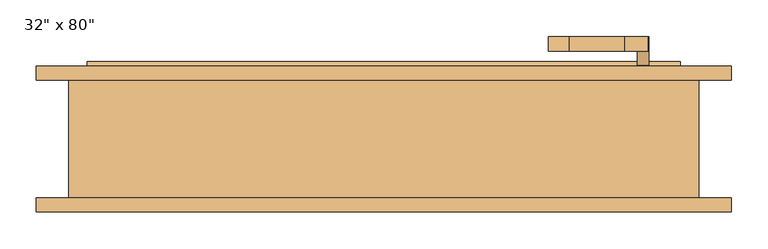
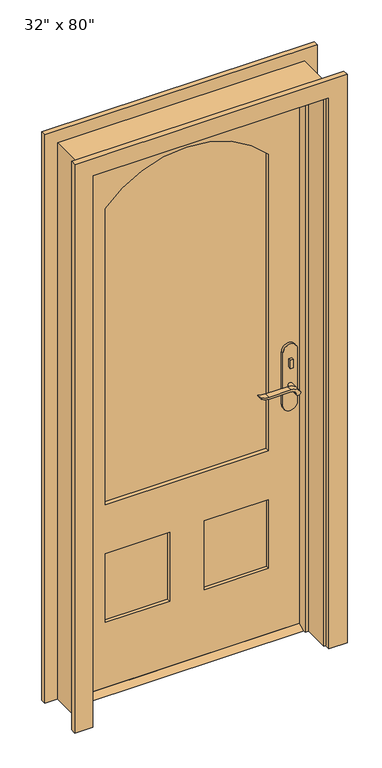
"""IFC4 building model written with IfcOpenShell, lengths in millimetres: door geometry."""

import ifcopenshell
import ifcopenshell.guid

model = None  # the IFC model being written
_history = None  # IfcOwnerHistory: only IFC2X3 demands one
_inside = {}  # id of a spatial element -> (the spatial element, [elements in it])
_under = {}  # id of a project, library or spatial element -> (it, [spatial elements below it])
_declared = {}  # id of a project -> (the project, [libraries it declares])
_typed = {}  # id of a type object -> (the type object, [elements of that type])
_made_of = {}  # id of a material, layer set ... -> (it, [elements and type objects made of it])


def new_model(schema):
    """Start an empty IFC model of exactly this schema.

    Asked for "IFC4X3", IfcOpenShell would pick the latest addendum, in which some entities
    have other attributes; the version numbers below select the first issue.
    IFC2X3 requires an IfcOwnerHistory on every rooted entity: one is made here for all.
    """
    global model, _history
    if schema == "IFC4X3":
        model = ifcopenshell.file(schema_version=(4, 3, 0, 0))
    else:
        model = ifcopenshell.file(schema=schema)
    _inside.clear()
    _under.clear()
    _declared.clear()
    _typed.clear()
    _made_of.clear()
    _history = None
    if model.schema == "IFC2X3":
        org = make("IfcOrganization", Name="unknown")
        user = make(
            "IfcPersonAndOrganization",
            ThePerson=make("IfcPerson", FamilyName="unknown"),
            TheOrganization=org,
        )
        app = make(
            "IfcApplication",
            ApplicationDeveloper=org,
            Version="unknown",
            ApplicationFullName="unknown",
            ApplicationIdentifier="unknown",
        )
        _history = make(
            "IfcOwnerHistory",
            OwningUser=user,
            OwningApplication=app,
            ChangeAction="ADDED",
            CreationDate=0,
        )
    return model


def make(cls, **values):
    """One entity of the class cls with the attributes given. An attribute that is None is left unset."""
    return model.create_entity(
        cls, **{name: value for name, value in values.items() if value is not None}
    )


def rooted(cls, **values):
    """An entity with a GlobalId (a new one), such as an element, a storey or a relation."""
    return make(cls, GlobalId=ifcopenshell.guid.new(), OwnerHistory=_history, **values)


def si_unit(unit_type, name, prefix=None):
    """IfcSIUnit, for example si_unit("LENGTHUNIT", "METRE", prefix="MILLI")."""
    return make("IfcSIUnit", UnitType=unit_type, Prefix=prefix, Name=name)


def assignment(units):
    """IfcUnitAssignment: the units of a project."""
    return None if units is None else make("IfcUnitAssignment", Units=units)


def point(xyz):
    """IfcCartesianPoint."""
    return None if xyz is None else make("IfcCartesianPoint", Coordinates=xyz)


def direction(xyz):
    """IfcDirection."""
    return None if xyz is None else make("IfcDirection", DirectionRatios=xyz)


def frame(location, z_axis=None, x_axis=None):
    """IfcAxis2Placement3D, a coordinate frame: its origin and axes. An axis left out is left unset."""
    return make(
        "IfcAxis2Placement3D",
        Location=point(location),
        Axis=direction(z_axis),
        RefDirection=direction(x_axis),
    )


def frame_2d(location, x_axis=None):
    """IfcAxis2Placement2D, a coordinate frame in the plane: its origin and x axis."""
    return make(
        "IfcAxis2Placement2D", Location=point(location), RefDirection=direction(x_axis)
    )


def origin():
    """The frame at (0, 0, 0) with its axes left unset."""
    return frame((0.0, 0.0, 0.0))


def place(relative_to, where):
    """IfcLocalPlacement: puts the frame where relative to a parent placement (None: the world)."""
    return make(
        "IfcLocalPlacement", PlacementRelTo=relative_to, RelativePlacement=where
    )


def context(
    kind, dimensions, precision=None, world=None, true_north=None, identifier=None
):
    """IfcGeometricRepresentationContext, for example the 3D "Model" context."""
    return make(
        "IfcGeometricRepresentationContext",
        ContextIdentifier=identifier,
        ContextType=kind,
        CoordinateSpaceDimension=dimensions,
        Precision=precision,
        WorldCoordinateSystem=world,
        TrueNorth=true_north,
    )


def project(units=None, contexts=None):
    """IfcProject with its units and contexts."""
    return rooted(
        "IfcProject",
        Name="project",
        RepresentationContexts=contexts,
        UnitsInContext=assignment(units),
    )


def spatial(cls, under=None, at=None, **own):
    """A site, building, storey or space (cls), placed at a placement, below another one or the project."""
    s = rooted(cls, ObjectPlacement=at, **own)
    if under is not None:
        _under.setdefault(under.id(), (under, []))[1].append(s)
    return s


def polyline(points):
    """IfcPolyline through the points."""
    return make("IfcPolyline", Points=[point(p) for p in points])


def circle_curve(where, radius):
    """IfcCircle in the frame where."""
    return make("IfcCircle", Position=where, Radius=radius)


def trimmed(basis, trim1, trim2, sense, master):
    """IfcTrimmedCurve: the piece of a basis curve between two trims."""
    return make(
        "IfcTrimmedCurve",
        BasisCurve=basis,
        Trim1=trim1,
        Trim2=trim2,
        SenseAgreement=sense,
        MasterRepresentation=master,
    )


def segment(curve, same_sense, transition):
    """IfcCompositeCurveSegment."""
    return make(
        "IfcCompositeCurveSegment",
        Transition=transition,
        SameSense=same_sense,
        ParentCurve=curve,
    )


def composite_curve(segments, self_intersect=None):
    """IfcCompositeCurve: segments joined end to end."""
    return make("IfcCompositeCurve", Segments=segments, SelfIntersect=self_intersect)


def outline(outer, holes=None, kind="AREA"):
    """IfcArbitraryClosedProfileDef: a profile drawn as a closed curve; with holes, ...WithVoids."""
    if holes is None:
        return make("IfcArbitraryClosedProfileDef", ProfileType=kind, OuterCurve=outer)
    return make(
        "IfcArbitraryProfileDefWithVoids",
        ProfileType=kind,
        OuterCurve=outer,
        InnerCurves=holes,
    )


def extrude(swept, where, along, depth):
    """IfcExtrudedAreaSolid: the profile swept, set in the frame where, extruded along a direction by depth."""
    return make(
        "IfcExtrudedAreaSolid",
        SweptArea=swept,
        Position=where,
        ExtrudedDirection=direction(along),
        Depth=depth,
    )


def faces_of(points, faces, orient=None, outer=None):
    """IfcFace entities. A face is a list of loops; a loop is a list of indices into points, from 0.

    orient and outer hold one flag for each loop. By default every Orientation is true, the
    first loop of a face is its IfcFaceOuterBound and the others are IfcFaceBound.
    """
    made = []
    for i, loops in enumerate(faces):
        bounds = []
        for j, loop in enumerate(loops):
            is_outer = j == 0 if outer is None else outer[i][j]
            bounds.append(
                make(
                    "IfcFaceOuterBound" if is_outer else "IfcFaceBound",
                    Bound=make("IfcPolyLoop", Polygon=[points[k] for k in loop]),
                    Orientation=True if orient is None else orient[i][j],
                )
            )
        made.append(make("IfcFace", Bounds=bounds))
    return made


def faceted_brep(points, faces, orient=None, outer=None, voids=None):
    """IfcFacetedBrep: a solid bounded by flat faces; with voids (closed shells), ...WithVoids."""
    shared = [point(p) for p in points]
    hull = make("IfcClosedShell", CfsFaces=faces_of(shared, faces, orient, outer))
    if voids is None:
        return make("IfcFacetedBrep", Outer=hull)
    return make(
        "IfcFacetedBrepWithVoids",
        Outer=hull,
        Voids=[
            make(cls, CfsFaces=faces_of(shared, fs, o, b)) for cls, fs, o, b in voids
        ],
    )


def shape(context_of_items, identifier, shape_type, items):
    """IfcShapeRepresentation: the items that make up one representation, for example the "Body"."""
    return make(
        "IfcShapeRepresentation",
        ContextOfItems=context_of_items,
        RepresentationIdentifier=identifier,
        RepresentationType=shape_type,
        Items=items,
    )


def source(mapping_origin, context_of_items, identifier, shape_type, items):
    """IfcRepresentationMap: a shape defined once, which mapped items show again and again."""
    return make(
        "IfcRepresentationMap",
        MappingOrigin=mapping_origin,
        MappedRepresentation=shape(context_of_items, identifier, shape_type, items),
    )


def transform(
    local_origin,
    x_axis=None,
    y_axis=None,
    z_axis=None,
    scale=None,
    scale2=None,
    scale3=None,
    uniform=True,
):
    """IfcCartesianTransformationOperator3D, or its non-uniform kind. x_axis, y_axis, z_axis: its Axis1, 2, 3."""
    if uniform:
        return make(
            "IfcCartesianTransformationOperator3D",
            Axis1=direction(x_axis),
            Axis2=direction(y_axis),
            LocalOrigin=point(local_origin),
            Scale=scale,
            Axis3=direction(z_axis),
        )
    return make(
        "IfcCartesianTransformationOperator3DnonUniform",
        Axis1=direction(x_axis),
        Axis2=direction(y_axis),
        LocalOrigin=point(local_origin),
        Scale=scale,
        Axis3=direction(z_axis),
        Scale2=scale2,
        Scale3=scale3,
    )


def mapped(mapping_source, mapping_target):
    """IfcMappedItem: shows the shape of a source again, moved by a transform."""
    return make(
        "IfcMappedItem", MappingSource=mapping_source, MappingTarget=mapping_target
    )


def made_of(thing, what):
    """Note that an element or type object is made of a material, layer set ...; save() writes the relation."""
    if what is not None:
        _made_of.setdefault(what.id(), (what, []))[1].append(thing)
    return thing


def element(
    cls,
    number,
    at=None,
    inside=None,
    cuts=None,
    type_object=None,
    material=None,
    context=None,
    identifier="Body",
    shape_type=None,
    held_by="IfcProductDefinitionShape",
    body=None,
    shapes=None,
    **own,
):
    """One element of the class cls, such as IfcWall. Its Tag is "e" and its number.

    at: its placement. inside: the storey or other place that contains it. cuts: it is an
    opening in that element (IfcRelVoidsElement). A single representation is given by context,
    identifier, shape_type and body (its items); several are given by shapes. held_by: the class
    of the entity that holds the representations. save() writes the other relations.
    """
    e = rooted(cls, Tag="e%d" % number, ObjectPlacement=at, **own)
    if body is not None:
        shapes = [shape(context, identifier, shape_type, body)]
    if shapes is not None:
        e.Representation = make(held_by, Representations=shapes)
    if inside is not None:
        _inside.setdefault(inside.id(), (inside, []))[1].append(e)
    if cuts is not None:
        rooted(
            "IfcRelVoidsElement", RelatingBuildingElement=cuts, RelatedOpeningElement=e
        )
    if type_object is not None:
        _typed.setdefault(type_object.id(), (type_object, []))[1].append(e)
    return made_of(e, material)


def aggregate(whole, parts):
    """IfcRelAggregates: a whole, such as a stair, and the parts it consists of."""
    return rooted("IfcRelAggregates", RelatingObject=whole, RelatedObjects=parts)


def save(model, path):
    """Write the relations noted so far, then the file.

    IfcRelAggregates (storeys below a building ...), IfcRelContainedInSpatialStructure (elements
    in a storey), IfcRelDefinesByType, IfcRelAssociatesMaterial and IfcRelDeclares: one each for
    every whole, place, type object, material and project.
    """
    for whole, parts in _under.values():
        aggregate(whole, parts)
    for where, things in _inside.values():
        rooted(
            "IfcRelContainedInSpatialStructure",
            RelatedElements=things,
            RelatingStructure=where,
        )
    for kind, things in _typed.values():
        rooted("IfcRelDefinesByType", RelatedObjects=things, RelatingType=kind)
    for what, things in _made_of.values():
        rooted("IfcRelAssociatesMaterial", RelatedObjects=things, RelatingMaterial=what)
    for by, libraries in _declared.values():
        rooted("IfcRelDeclares", RelatingContext=by, RelatedDefinitions=libraries)
    model.write(path)


def door_3993ae6d(model_context):
    return source(origin(), model_context, "Body", "SolidModel", [
        extrude(outline(polyline([(42.8625, 12.7), (77.7875, 12.7), (103.1875, 0.0), (17.4625, 0.0), (42.8625, 12.7)])), frame((-406.4, 0.0, 0.0), z_axis=(1.0, 0.0, 0.0), x_axis=(0.0, 1.0, 0.0)), (0.0, 0.0, 1.0), 812.8),
        extrude(outline(polyline([(360.6, 22.8625), (350.6, 22.8625), (350.6, 32.8625), (360.6, 32.8625), (360.6, 22.8625)])), frame((0.0, 0.0, 981.9), z_axis=(0.0, 0.0, 1.0), x_axis=(1.0, 0.0, 0.0)), (0.0, 0.0, 1.0), 30.0),
        extrude(outline(composite_curve([segment(trimmed(circle_curve(frame_2d((996.9, 355.6)), 8.0), [point((996.9, 347.6))], [point((996.9, 363.6))], False, "CARTESIAN"), True, "CONTINUOUS"), segment(trimmed(circle_curve(frame_2d((996.9, 355.6)), 8.0), [point((996.9, 363.6))], [point((996.9, 347.6))], False, "CARTESIAN"), True, "CONTINUOUS")], self_intersect=False)), frame((0.0, 87.7875, 0.0), z_axis=(0.0, 1.0, 0.0), x_axis=(0.0, 0.0, 1.0)), (0.0, 0.0, 1.0), 10.0),
        extrude(outline(composite_curve([segment(trimmed(circle_curve(frame_2d((897.1555521, 331.9324871)), 37.2832219), [point((919.0523287, 362.1081363))], [point((934.4, 330.2325667))], False, "CARTESIAN"), True, "CONTINUOUS"), segment(polyline([(934.4, 330.2325667), (934.4, 253.9564091)]), True, "CONTINUOUS"), segment(trimmed(circle_curve(frame_2d((1017.6850638, 254.0227909)), 83.2850902), [point((934.4, 253.9564091))], [point((939.4, 225.6))], True, "CARTESIAN"), True, "CONTINUOUS"), segment(polyline([(939.4, 225.6), (936.6135558, 225.6)]), True, "CONTINUOUS"), segment(trimmed(circle_curve(frame_2d((986.6709207, 257.5396612)), 59.3791355), [point((936.6135558, 225.6))], [point((927.4, 253.9564091))], False, "CARTESIAN"), True, "CONTINUOUS"), segment(polyline([(927.4, 253.9564091), (927.4, 330.2138099)]), True, "CONTINUOUS"), segment(trimmed(circle_curve(frame_2d((909.2738613, 330.2138099)), 18.1261387), [point((927.4, 330.2138099))], [point((914.4, 347.6))], True, "CARTESIAN"), True, "CONTINUOUS"), segment(trimmed(circle_curve(frame_2d((914.4, 355.6)), 8.0), [point((914.4, 347.6))], [point((919.0523287, 362.1081363))], False, "CARTESIAN"), True, "CONTINUOUS")], self_intersect=False)), frame((0.0, -17.1375, 0.0), z_axis=(0.0, 1.0, 0.0), x_axis=(0.0, 0.0, 1.0)), (0.0, 0.0, 1.0), 20.0),
        extrude(outline(composite_curve([segment(trimmed(circle_curve(frame_2d((914.4, 355.6)), 8.0), [point((914.3999903, 347.6))], [point((919.0523287, 362.1081363))], False, "CARTESIAN"), True, "CONTINUOUS"), segment(trimmed(circle_curve(frame_2d((897.1555521, 331.9324871)), 37.2832219), [point((919.0523287, 362.1081363))], [point((934.4, 330.2325667))], False, "CARTESIAN"), True, "CONTINUOUS"), segment(polyline([(934.4, 330.2325667), (934.4, 253.9564091)]), True, "CONTINUOUS"), segment(trimmed(circle_curve(frame_2d((1017.6850638, 254.0227909)), 83.2850902), [point((934.4, 253.9564091))], [point((939.4, 225.6))], True, "CARTESIAN"), True, "CONTINUOUS"), segment(polyline([(939.4, 225.6), (936.6135558, 225.6)]), True, "CONTINUOUS"), segment(trimmed(circle_curve(frame_2d((986.6709207, 257.5396612)), 59.3791355), [point((936.6135558, 225.6))], [point((927.4, 253.9564091))], False, "CARTESIAN"), True, "CONTINUOUS"), segment(polyline([(927.4, 253.9564091), (927.4, 330.2138122)]), True, "CONTINUOUS"), segment(trimmed(circle_curve(frame_2d((909.2738682, 330.2138122)), 18.1261318), [point((927.4, 330.2138122))], [point((914.3999903, 347.6))], True, "CARTESIAN"), True, "CONTINUOUS")], self_intersect=False)), frame((0.0, 117.7875, 0.0), z_axis=(0.0, 1.0, 0.0), x_axis=(0.0, 0.0, 1.0)), (0.0, 0.0, 1.0), 20.0),
        extrude(outline(composite_curve([segment(trimmed(circle_curve(frame_2d((914.4, 355.6)), 8.0), [point((914.4, 347.6))], [point((914.4, 363.6))], False, "CARTESIAN"), True, "CONTINUOUS"), segment(trimmed(circle_curve(frame_2d((914.4, 355.6)), 8.0), [point((914.4, 363.6))], [point((914.4, 347.6))], False, "CARTESIAN"), True, "CONTINUOUS")], self_intersect=False)), frame((0.0, 2.8625, 0.0), z_axis=(0.0, 1.0, 0.0), x_axis=(0.0, 0.0, 1.0)), (0.0, 0.0, 1.0), 30.0),
        extrude(outline(composite_curve([segment(trimmed(circle_curve(frame_2d((914.4, 355.6)), 8.0), [point((914.4, 347.6))], [point((914.4, 363.6))], False, "CARTESIAN"), True, "CONTINUOUS"), segment(trimmed(circle_curve(frame_2d((914.4, 355.6)), 8.0), [point((914.4, 363.6))], [point((914.4, 347.6))], False, "CARTESIAN"), True, "CONTINUOUS")], self_intersect=False)), frame((0.0, 87.7875, 0.0), z_axis=(0.0, 1.0, 0.0), x_axis=(0.0, 0.0, 1.0)), (0.0, 0.0, 1.0), 30.0),
        extrude(outline(composite_curve([segment(polyline([(844.4, 380.6), (1039.4, 380.6)]), True, "CONTINUOUS"), segment(trimmed(circle_curve(frame_2d((1039.4, 355.6)), 25.0), [point((1039.4, 380.6))], [point((1039.4, 330.6))], False, "CARTESIAN"), True, "CONTINUOUS"), segment(polyline([(1039.4, 330.6), (844.4, 330.6)]), True, "CONTINUOUS"), segment(trimmed(circle_curve(frame_2d((844.4, 355.6)), 25.0), [point((844.4, 330.6))], [point((844.4, 380.6))], False, "CARTESIAN"), True, "CONTINUOUS")], self_intersect=False)), frame((0.0, 32.8625, 0.0), z_axis=(0.0, 1.0, 0.0), x_axis=(0.0, 0.0, 1.0)), (0.0, 0.0, 1.0), 10.0),
        extrude(outline(composite_curve([segment(polyline([(844.4, 380.6), (1039.4, 380.6)]), True, "CONTINUOUS"), segment(trimmed(circle_curve(frame_2d((1039.4, 355.6)), 25.0), [point((1039.4, 380.6))], [point((1039.4, 330.6))], False, "CARTESIAN"), True, "CONTINUOUS"), segment(polyline([(1039.4, 330.6), (844.4, 330.6)]), True, "CONTINUOUS"), segment(trimmed(circle_curve(frame_2d((844.4, 355.6)), 25.0), [point((844.4, 330.6))], [point((844.4, 380.6))], False, "CARTESIAN"), True, "CONTINUOUS")], self_intersect=False)), frame((0.0, 77.7875, 0.0), z_axis=(0.0, 1.0, 0.0), x_axis=(0.0, 0.0, 1.0)), (0.0, 0.0, 1.0), 10.0),
        extrude(outline(polyline([(2032.0, -406.4), (12.7, -406.4), (12.7, 406.4), (2032.0, 406.4), (2032.0, -406.4)]), holes=[composite_curve([segment(polyline([(688.975, -285.75), (1784.35, -285.75)]), True, "CONTINUOUS"), segment(trimmed(circle_curve(frame_2d((1526.38125, 0.0)), 384.96875), [point((1784.35, -285.75))], [point((1784.35, 285.75))], True, "CARTESIAN"), True, "CONTINUOUS"), segment(polyline([(1784.35, 285.75), (688.975, 285.75), (688.975, -285.75)]), True, "CONTINUOUS")], self_intersect=False), polyline([(508.0, -60.325), (254.0, -60.325), (254.0, -285.75), (508.0, -285.75), (508.0, -60.325)]), polyline([(508.0, 285.75), (254.0, 285.75), (254.0, 60.325), (508.0, 60.325), (508.0, 285.75)])]), frame((0.0, 42.8625, 0.0), z_axis=(0.0, 1.0, 0.0), x_axis=(0.0, 0.0, 1.0)), (0.0, 0.0, 1.0), 34.925),
        faceted_brep([(431.8, 77.7875, 0.0), (431.8, -84.1375, 0.0), (406.4, -84.1375, 0.0), (406.4, 7.9375, 0.0), (393.7, 7.9375, 0.0), (393.7, 42.8625, 0.0), (406.4, 42.8625, 0.0), (406.4, 77.7875, 0.0), (431.8, 77.7875, 2057.4), (431.8, -84.1375, 2057.4), (-431.8, -84.1375, 2057.4), (-431.8, -84.1375, 0.0), (-406.4, -84.1375, 0.0), (-406.4, -84.1375, 2032.0), (406.4, -84.1375, 2032.0), (406.4, 7.9375, 2032.0), (-406.4, 7.9375, 2032.0), (-406.4, 7.9375, 0.0), (-393.7, 7.9375, 0.0), (-393.7, 7.9375, 2019.3), (393.7, 7.9375, 2019.3), (393.7, 42.8625, 2019.3), (-393.7, 42.8625, 2019.3), (-393.7, 42.8625, 0.0), (-406.4, 42.8625, 0.0), (-406.4, 42.8625, 2032.0), (406.4, 42.8625, 2032.0), (406.4, 77.7875, 2032.0), (-406.4, 77.7875, 2032.0), (-406.4, 77.7875, 0.0), (-431.8, 77.7875, 0.0), (-431.8, 77.7875, 2057.4)], [[[0, 1, 2, 3, 4, 5, 6, 7]], [[1, 0, 8, 9]], [[2, 1, 9, 10, 11, 12, 13, 14]], [[3, 2, 14, 15]], [[4, 3, 15, 16, 17, 18, 19, 20]], [[5, 4, 20, 21]], [[6, 5, 21, 22, 23, 24, 25, 26]], [[7, 6, 26, 27]], [[0, 7, 27, 28, 29, 30, 31, 8]], [[9, 8, 31, 10]], [[15, 14, 13, 16]], [[21, 20, 19, 22]], [[27, 26, 25, 28]], [[30, 29, 24, 23, 18, 17, 12, 11]], [[10, 31, 30, 11]], [[16, 13, 12, 17]], [[22, 19, 18, 23]], [[28, 25, 24, 29]]]),
        extrude(outline(polyline([(-60.325, 54.5041667), (-285.75, 54.5041667), (-285.75, 66.1458333), (-60.325, 66.1458333), (-60.325, 54.5041667)])), frame((0.0, 0.0, 254.0), z_axis=(0.0, 0.0, 1.0), x_axis=(1.0, 0.0, 0.0)), (0.0, 0.0, 1.0), 254.0),
        extrude(outline(polyline([(285.75, 54.5041667), (60.325, 54.5041667), (60.325, 66.1458333), (285.75, 66.1458333), (285.75, 54.5041667)])), frame((0.0, 0.0, 254.0), z_axis=(0.0, 0.0, 1.0), x_axis=(1.0, 0.0, 0.0)), (0.0, 0.0, 1.0), 254.0),
        extrude(outline(composite_curve([segment(polyline([(688.975, -285.75), (688.975, 285.75), (1784.35, 285.75)]), True, "CONTINUOUS"), segment(trimmed(circle_curve(frame_2d((1526.38125, 0.0)), 384.96875), [point((1784.35, 285.75))], [point((1784.35, -285.75))], False, "CARTESIAN"), True, "CONTINUOUS"), segment(polyline([(1784.35, -285.75), (688.975, -285.75)]), True, "CONTINUOUS")], self_intersect=False)), frame((0.0, 56.8325, 0.0), z_axis=(0.0, 1.0, 0.0), x_axis=(0.0, 0.0, 1.0)), (0.0, 0.0, 1.0), 6.985),
        extrude(outline(polyline([(0.0, -476.25), (0.0, -412.75), (2038.35, -412.75), (2038.35, 412.75), (0.0, 412.75), (0.0, 476.25), (2101.85, 476.25), (2101.85, -476.25), (0.0, -476.25)])), frame((0.0, -103.1875, 0.0), z_axis=(0.0, 1.0, 0.0), x_axis=(0.0, 0.0, 1.0)), (0.0, 0.0, 1.0), 19.05),
        extrude(outline(polyline([(0.0, -476.25), (0.0, -412.75), (2038.35, -412.75), (2038.35, 412.75), (0.0, 412.75), (0.0, 476.25), (2101.85, 476.25), (2101.85, -476.25), (0.0, -476.25)])), frame((0.0, 77.7875, 0.0), z_axis=(0.0, 1.0, 0.0), x_axis=(0.0, 0.0, 1.0)), (0.0, 0.0, 1.0), 19.05),
    ])


if __name__ == "__main__":
    model = new_model("IFC4")
    model_context = context("Model", 3, world=origin())
    ifc_project = project(units=[si_unit("LENGTHUNIT", "METRE", prefix="MILLI")], contexts=[model_context])
    site = spatial("IfcSite", under=ifc_project)
    building = spatial("IfcBuilding", under=site)
    placement = place(None, origin())
    door_shape = door_3993ae6d(model_context)
    element("IfcDoor", 1, ObjectType="Door-Exterior-Single-Entry-Half Arch Glass-Wood_Clad : 32\" x 80\"", at=placement, inside=building, context=model_context, shape_type="MappedRepresentation", body=[
        mapped(door_shape, transform((0.0, 0.0, 0.0), x_axis=(1.0, 0.0, 0.0), y_axis=(0.0, 1.0, 0.0), z_axis=(0.0, 0.0, 1.0))),
    ])
    save(model, "model.ifc")

# Revit data of these elements
# Type "Door-Exterior-Single-Entry-Half Arch Glass-Wood_Clad : 32\" x 80\""
#   Type Mark = "112"
#   COBie.Type.CreatedBy = "doug.wood@us.ibm.com"
#   COBie.Type.CreatedOn = "2016-04-14T02:07:24"
#   COBie.Type.Name = "Doors_Door-Exterior-Single-Entry-Half Arch Glass-Wood_Clad_32\" x 80\"_112"
#   COBie.Type.Category = "23-30 10 14 : Passage Doors by Material"
#   COBie.Type.Description = "Door-Exterior-Single-Entry-Half Arch Glass-Wood_Clad_32\" x 80\""
#   COBie.Type.Manufacturer = ""
#   COBie.Type.ModelNumber = ""
#   Assembly Code = "B2030100"
#   Analytic Construction = "French door, wood frame with single glass"
#   COBie.Type.ReplacementCost = 0
#   Threshold Offset [instance default] = 0' - 0 1/2"
#   Thickness = 0' - 1 3/8"
#   Thermal Resistance (R) = 0.188367 (m²·K)/W
#   Swing Angle [instance default] = 90.00°
#   Stiles = 0' - 4 3/4"
#   Rough Width = 2' - 10"
#   Rough Height = 6' - 9"
#   Radius = 1' - 3 5/32"
#   Lock Rail = 0' - 7 1/8"
#   Height = 6' - 8"
#   Width = 2' - 8"
#   Heat Transfer Coefficient (U) = 5.30918 W/(m²·K)
#   Door Offset [instance default] = 0' - 0"
#   Bottom Rail = 0' - 9 1/2"
#   COBie.Type = no
#   Threshold [instance default] = yes
#   Function = 1
#   Exterior Trim [instance default] = yes
#   Trim Material = Trim - White
#   Threshold Material = Trim - White
#   Panel Material = Paint - Dark Blue
#   Glazing = Glass
#   Frame Material = Door - Panel - White
#   Door Handle Material = ARCAT - Metal - Brass, Polished
#   Visual Light Transmittance = 0
#   Solar Heat Gain Coefficient = 0
#   Wall Closure = (empty or 0)
#   Construction Type = (empty or 0)
# Element 1 (IfcDoor, "Door-Exterior-Single-Entry-Half Arch Glass-Wood_Clad : 32\" x 80\"")
#   Materials on its faces: "ARCAT - Metal - Brass, Polished", "Paint - Dark Blue", "Trim - White", "Door - Panel - White", "Glass"
# Materials
#   "Trim - White": class "Wood", colour RGB 255 255 255, transparency 0, Cost = 0
#   "Paint - Dark Blue": class "Paint", colour RGB 29 38 150, transparency 0, Description = "Paint - Dark Blue", Cost = 0
#   "Glass": class "Glass", colour RGB 0 128 192, transparency 0.75, Description = "Soda Lime Glass", Cost = 0
#   "Door - Panel - White": class "Wood", colour RGB 255 255 255, transparency 0, Cost = 0
#   "ARCAT - Metal - Brass, Polished": class "Unassigned", colour RGB 246 240 166, transparency 0, Keynote = "05050", Model = "Generic", Manufacturer = "Generic", Description = "Steel, Chrome Plated"
